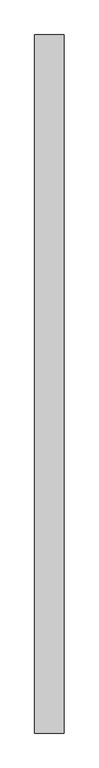
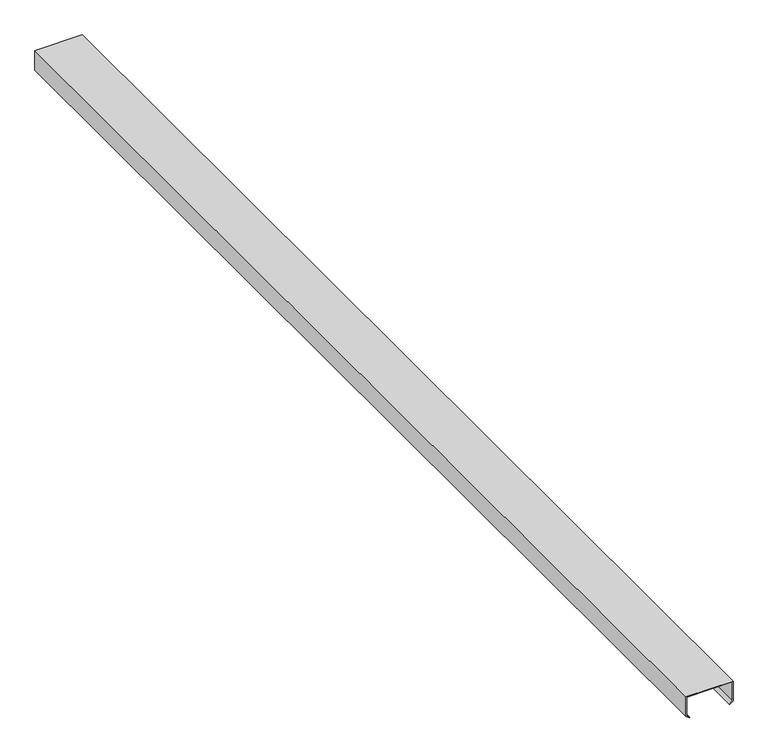
"""IFC4 building model written with IfcOpenShell, lengths in millimetres: proxy geometry, Generic Models 7:Generic Models 1:1:Generic Models 1:1 : Generic Models 7:Generic Models 1:337419:18 : Generic Models 7:Generic Models 1:1:Generic Models 1:1 : Generic Models 7:Generic Models 1:337419:306201."""

from ifc_helpers import new_model, si_unit, frame, origin, place, context, project, spatial, polyline, outline, extrude, source, transform, mapped, element, save


def generic_models_6bc2a326(model_context):
    return source(origin(), model_context, "Body", "SweptSolid", [
        extrude(outline(polyline([(4985.940625, 579307.711724), (4985.940625, 579104.511724), (4897.040625, 579104.511724), (4884.7955211, 579119.1048707), (4886.9236883, 579120.890615), (4898.336086, 579107.289849), (4983.1625, 579107.289849), (4983.1625, 579304.933599), (4898.336086, 579304.933599), (4886.9236883, 579291.3328331), (4884.7955211, 579293.1185774), (4897.040625, 579307.711724), (4985.940625, 579307.711724)])), frame((0.0, -578797.4913841, 0.0), z_axis=(0.0, 1.0, 0.0), x_axis=(0.0, 0.0, 1.0)), (0.0, 0.0, 1.0), 4854.575),
    ])


if __name__ == "__main__":
    model = new_model("IFC4")
    model_context = context("Model", 3, world=origin())
    ifc_project = project(units=[si_unit("LENGTHUNIT", "METRE", prefix="MILLI")], contexts=[model_context])
    site = spatial("IfcSite", under=ifc_project)
    building = spatial("IfcBuilding", under=site)
    placement = place(None, origin())
    generic_models_shape = generic_models_6bc2a326(model_context)
    element("IfcBuildingElementProxy", 1, Name="Generic Models 7:Generic Models 1:1:Generic Models 1:1 : Generic Models 7:Generic Models 1:337419:18 : Generic Models 7:Generic Models 1:1:Generic Models 1:1 : Generic Models 7:Generic Models 1:337419:306201", ObjectType="Generic Models 7:Generic Models 1:1:Generic Models 1:1 : Generic Models 7:Generic Models 1:337419:18 : Generic Models 7:Generic Models 1:1:Generic Models 1:1 : Generic Models 7:Generic Models 1:337419:306201", at=placement, inside=building, context=model_context, shape_type="MappedRepresentation", body=[
        mapped(generic_models_shape, transform((0.0, 0.0, 0.0), x_axis=(1.0, 0.0, 0.0), y_axis=(0.0, 1.0, 0.0), z_axis=(0.0, 0.0, 1.0))),
    ])
    save(model, "model.ifc")

# Revit data of these elements
# Type "Generic Models 7:Generic Models 1:1:Generic Models 1:1 : Generic Models 7:Generic Models 1:337419:18 : Generic Models 7:Generic Models 1:1:Generic Models 1:1 : Generic Models 7:Generic Models 1:337419:306201"
#   NameOverride = "Generic Models 7:Generic Models 1:1:Generic Models 1:1 : Generic Models 7:Generic Models 1:337419:306201"
#   ObjectTypeOverride = "Generic Models 1:1 : Generic Models 7:Generic Models 1:337419"
#   Reference = "Generic Models 1"
#   Tag = "306201"
# Element 1 (IfcBuildingElementProxy, "Generic Models 7:Generic Models 1:1:Generic Models 1:1 : Generic Models 7:Generic Models 1:337419:18 : Generic Models 7:Generic Models 1:1:Generic Models 1:1 : Generic Models 7:Generic Models 1:337419:306201")
#   Materials on its faces: "'ZEE' SECTION (8.0x3.5Z - SEE STRUCT. DWGS)"
# Materials
#   "'ZEE' SECTION (8.0x3.5Z - SEE STRUCT. DWGS)": class "Unassigned", colour RGB 210 209 208, transparency 0, Keynote = "M05121300.02", Cost = 0
